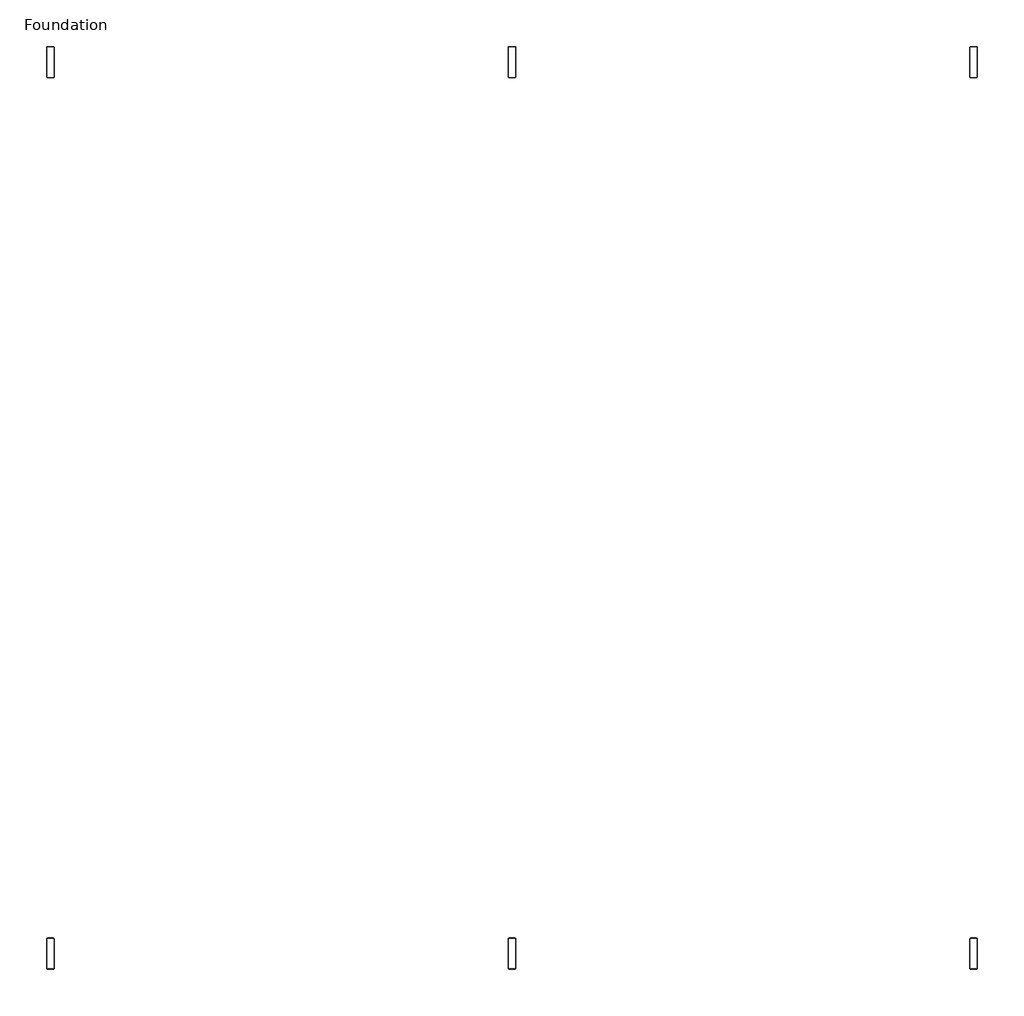
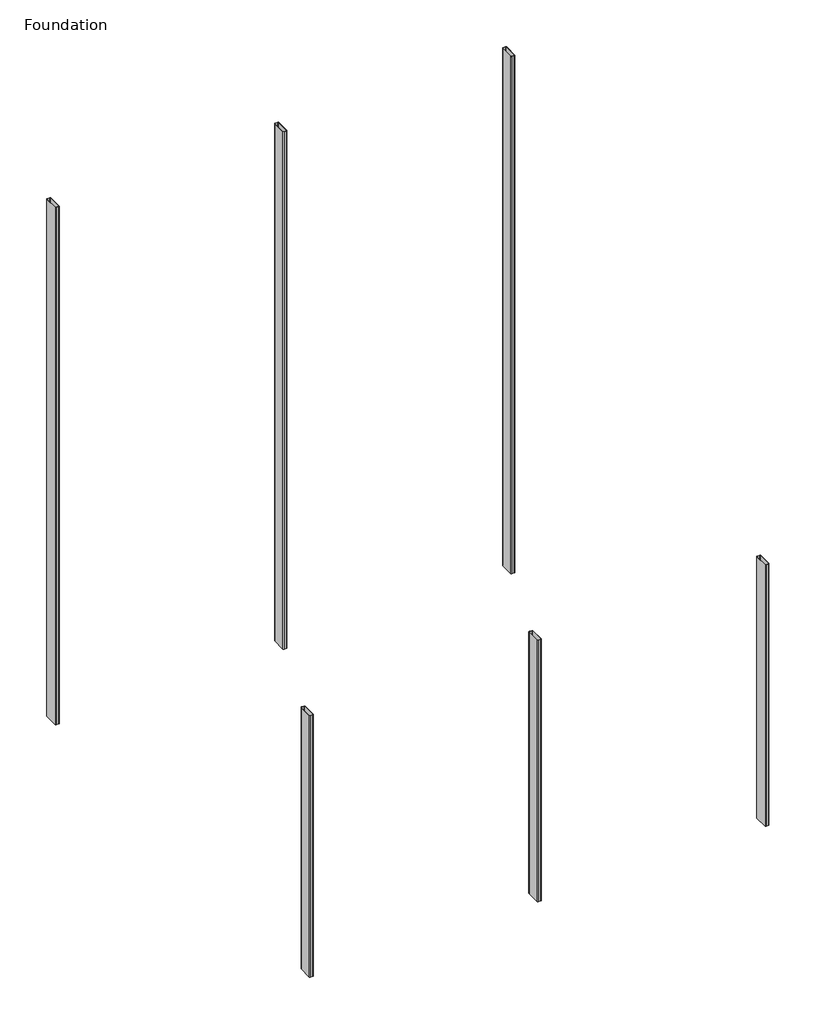
# One storey: 6 columns.
"""IFC4 building model written with IfcOpenShell, lengths in millimetres."""

import ifcopenshell
import ifcopenshell.guid

model = None  # the IFC model being written
_history = None  # IfcOwnerHistory: only IFC2X3 demands one
_inside = {}  # id of a spatial element -> (the spatial element, [elements in it])
_under = {}  # id of a project, library or spatial element -> (it, [spatial elements below it])
_declared = {}  # id of a project -> (the project, [libraries it declares])
_typed = {}  # id of a type object -> (the type object, [elements of that type])
_made_of = {}  # id of a material, layer set ... -> (it, [elements and type objects made of it])


def new_model(schema):
    """Start an empty IFC model of exactly this schema.

    Asked for "IFC4X3", IfcOpenShell would pick the latest addendum, in which some entities
    have other attributes; the version numbers below select the first issue.
    IFC2X3 requires an IfcOwnerHistory on every rooted entity: one is made here for all.
    """
    global model, _history
    if schema == "IFC4X3":
        model = ifcopenshell.file(schema_version=(4, 3, 0, 0))
    else:
        model = ifcopenshell.file(schema=schema)
    _inside.clear()
    _under.clear()
    _declared.clear()
    _typed.clear()
    _made_of.clear()
    _history = None
    if model.schema == "IFC2X3":
        org = make("IfcOrganization", Name="unknown")
        user = make(
            "IfcPersonAndOrganization",
            ThePerson=make("IfcPerson", FamilyName="unknown"),
            TheOrganization=org,
        )
        app = make(
            "IfcApplication",
            ApplicationDeveloper=org,
            Version="unknown",
            ApplicationFullName="unknown",
            ApplicationIdentifier="unknown",
        )
        _history = make(
            "IfcOwnerHistory",
            OwningUser=user,
            OwningApplication=app,
            ChangeAction="ADDED",
            CreationDate=0,
        )
    return model


def make(cls, **values):
    """One entity of the class cls with the attributes given. An attribute that is None is left unset."""
    return model.create_entity(
        cls, **{name: value for name, value in values.items() if value is not None}
    )


def rooted(cls, **values):
    """An entity with a GlobalId (a new one), such as an element, a storey or a relation."""
    return make(cls, GlobalId=ifcopenshell.guid.new(), OwnerHistory=_history, **values)


def si_unit(unit_type, name, prefix=None):
    """IfcSIUnit, for example si_unit("LENGTHUNIT", "METRE", prefix="MILLI")."""
    return make("IfcSIUnit", UnitType=unit_type, Prefix=prefix, Name=name)


def assignment(units):
    """IfcUnitAssignment: the units of a project."""
    return None if units is None else make("IfcUnitAssignment", Units=units)


def point(xyz):
    """IfcCartesianPoint."""
    return None if xyz is None else make("IfcCartesianPoint", Coordinates=xyz)


def direction(xyz):
    """IfcDirection."""
    return None if xyz is None else make("IfcDirection", DirectionRatios=xyz)


def frame(location, z_axis=None, x_axis=None):
    """IfcAxis2Placement3D, a coordinate frame: its origin and axes. An axis left out is left unset."""
    return make(
        "IfcAxis2Placement3D",
        Location=point(location),
        Axis=direction(z_axis),
        RefDirection=direction(x_axis),
    )


def frame_2d(location, x_axis=None):
    """IfcAxis2Placement2D, a coordinate frame in the plane: its origin and x axis."""
    return make(
        "IfcAxis2Placement2D", Location=point(location), RefDirection=direction(x_axis)
    )


def origin():
    """The frame at (0, 0, 0) with its axes left unset."""
    return frame((0.0, 0.0, 0.0))


def place(relative_to, where):
    """IfcLocalPlacement: puts the frame where relative to a parent placement (None: the world)."""
    return make(
        "IfcLocalPlacement", PlacementRelTo=relative_to, RelativePlacement=where
    )


def context(
    kind, dimensions, precision=None, world=None, true_north=None, identifier=None
):
    """IfcGeometricRepresentationContext, for example the 3D "Model" context."""
    return make(
        "IfcGeometricRepresentationContext",
        ContextIdentifier=identifier,
        ContextType=kind,
        CoordinateSpaceDimension=dimensions,
        Precision=precision,
        WorldCoordinateSystem=world,
        TrueNorth=true_north,
    )


def project(units=None, contexts=None):
    """IfcProject with its units and contexts."""
    return rooted(
        "IfcProject",
        Name="project",
        RepresentationContexts=contexts,
        UnitsInContext=assignment(units),
    )


def spatial(cls, under=None, at=None, **own):
    """A site, building, storey or space (cls), placed at a placement, below another one or the project."""
    s = rooted(cls, ObjectPlacement=at, **own)
    if under is not None:
        _under.setdefault(under.id(), (under, []))[1].append(s)
    return s


def polyline(points):
    """IfcPolyline through the points."""
    return make("IfcPolyline", Points=[point(p) for p in points])


def circle_curve(where, radius):
    """IfcCircle in the frame where."""
    return make("IfcCircle", Position=where, Radius=radius)


def trimmed(basis, trim1, trim2, sense, master):
    """IfcTrimmedCurve: the piece of a basis curve between two trims."""
    return make(
        "IfcTrimmedCurve",
        BasisCurve=basis,
        Trim1=trim1,
        Trim2=trim2,
        SenseAgreement=sense,
        MasterRepresentation=master,
    )


def segment(curve, same_sense, transition):
    """IfcCompositeCurveSegment."""
    return make(
        "IfcCompositeCurveSegment",
        Transition=transition,
        SameSense=same_sense,
        ParentCurve=curve,
    )


def composite_curve(segments, self_intersect=None):
    """IfcCompositeCurve: segments joined end to end."""
    return make("IfcCompositeCurve", Segments=segments, SelfIntersect=self_intersect)


def outline(outer, holes=None, kind="AREA"):
    """IfcArbitraryClosedProfileDef: a profile drawn as a closed curve; with holes, ...WithVoids."""
    if holes is None:
        return make("IfcArbitraryClosedProfileDef", ProfileType=kind, OuterCurve=outer)
    return make(
        "IfcArbitraryProfileDefWithVoids",
        ProfileType=kind,
        OuterCurve=outer,
        InnerCurves=holes,
    )


def extrude(swept, where, along, depth):
    """IfcExtrudedAreaSolid: the profile swept, set in the frame where, extruded along a direction by depth."""
    return make(
        "IfcExtrudedAreaSolid",
        SweptArea=swept,
        Position=where,
        ExtrudedDirection=direction(along),
        Depth=depth,
    )


def shape(context_of_items, identifier, shape_type, items):
    """IfcShapeRepresentation: the items that make up one representation, for example the "Body"."""
    return make(
        "IfcShapeRepresentation",
        ContextOfItems=context_of_items,
        RepresentationIdentifier=identifier,
        RepresentationType=shape_type,
        Items=items,
    )


def source(mapping_origin, context_of_items, identifier, shape_type, items):
    """IfcRepresentationMap: a shape defined once, which mapped items show again and again."""
    return make(
        "IfcRepresentationMap",
        MappingOrigin=mapping_origin,
        MappedRepresentation=shape(context_of_items, identifier, shape_type, items),
    )


def transform(
    local_origin,
    x_axis=None,
    y_axis=None,
    z_axis=None,
    scale=None,
    scale2=None,
    scale3=None,
    uniform=True,
):
    """IfcCartesianTransformationOperator3D, or its non-uniform kind. x_axis, y_axis, z_axis: its Axis1, 2, 3."""
    if uniform:
        return make(
            "IfcCartesianTransformationOperator3D",
            Axis1=direction(x_axis),
            Axis2=direction(y_axis),
            LocalOrigin=point(local_origin),
            Scale=scale,
            Axis3=direction(z_axis),
        )
    return make(
        "IfcCartesianTransformationOperator3DnonUniform",
        Axis1=direction(x_axis),
        Axis2=direction(y_axis),
        LocalOrigin=point(local_origin),
        Scale=scale,
        Axis3=direction(z_axis),
        Scale2=scale2,
        Scale3=scale3,
    )


def mapped(mapping_source, mapping_target):
    """IfcMappedItem: shows the shape of a source again, moved by a transform."""
    return make(
        "IfcMappedItem", MappingSource=mapping_source, MappingTarget=mapping_target
    )


def made_of(thing, what):
    """Note that an element or type object is made of a material, layer set ...; save() writes the relation."""
    if what is not None:
        _made_of.setdefault(what.id(), (what, []))[1].append(thing)
    return thing


def element(
    cls,
    number,
    at=None,
    inside=None,
    cuts=None,
    type_object=None,
    material=None,
    context=None,
    identifier="Body",
    shape_type=None,
    held_by="IfcProductDefinitionShape",
    body=None,
    shapes=None,
    **own,
):
    """One element of the class cls, such as IfcWall. Its Tag is "e" and its number.

    at: its placement. inside: the storey or other place that contains it. cuts: it is an
    opening in that element (IfcRelVoidsElement). A single representation is given by context,
    identifier, shape_type and body (its items); several are given by shapes. held_by: the class
    of the entity that holds the representations. save() writes the other relations.
    """
    e = rooted(cls, Tag="e%d" % number, ObjectPlacement=at, **own)
    if body is not None:
        shapes = [shape(context, identifier, shape_type, body)]
    if shapes is not None:
        e.Representation = make(held_by, Representations=shapes)
    if inside is not None:
        _inside.setdefault(inside.id(), (inside, []))[1].append(e)
    if cuts is not None:
        rooted(
            "IfcRelVoidsElement", RelatingBuildingElement=cuts, RelatedOpeningElement=e
        )
    if type_object is not None:
        _typed.setdefault(type_object.id(), (type_object, []))[1].append(e)
    return made_of(e, material)


def aggregate(whole, parts):
    """IfcRelAggregates: a whole, such as a stair, and the parts it consists of."""
    return rooted("IfcRelAggregates", RelatingObject=whole, RelatedObjects=parts)


def save(model, path):
    """Write the relations noted so far, then the file.

    IfcRelAggregates (storeys below a building ...), IfcRelContainedInSpatialStructure (elements
    in a storey), IfcRelDefinesByType, IfcRelAssociatesMaterial and IfcRelDeclares: one each for
    every whole, place, type object, material and project.
    """
    for whole, parts in _under.values():
        aggregate(whole, parts)
    for where, things in _inside.values():
        rooted(
            "IfcRelContainedInSpatialStructure",
            RelatedElements=things,
            RelatingStructure=where,
        )
    for kind, things in _typed.values():
        rooted("IfcRelDefinesByType", RelatedObjects=things, RelatingType=kind)
    for what, things in _made_of.values():
        rooted("IfcRelAssociatesMaterial", RelatedObjects=things, RelatingMaterial=what)
    for by, libraries in _declared.values():
        rooted("IfcRelDeclares", RelatingContext=by, RelatedDefinitions=libraries)
    model.write(path)


def hss_hollow_structural_section_column_hss8x2x3_16_e881e9b5(model_context):
    return source(origin(), model_context, "Body", "SweptSolid", [
        extrude(outline(composite_curve([segment(trimmed(circle_curve(frame_2d((16.5608, 92.7608)), 8.8392), [point((16.5608, 101.6))], [point((25.4, 92.7608))], False, "CARTESIAN"), True, "CONTINUOUS"), segment(polyline([(25.4, 92.7608), (25.4, -92.7608)]), True, "CONTINUOUS"), segment(trimmed(circle_curve(frame_2d((16.5608, -92.7608)), 8.8392), [point((25.4, -92.7608))], [point((16.5608, -101.6))], False, "CARTESIAN"), True, "CONTINUOUS"), segment(polyline([(16.5608, -101.6), (-16.5608, -101.6)]), True, "CONTINUOUS"), segment(trimmed(circle_curve(frame_2d((-16.5608, -92.7608)), 8.8392), [point((-16.5608, -101.6))], [point((-25.4, -92.7608))], False, "CARTESIAN"), True, "CONTINUOUS"), segment(polyline([(-25.4, -92.7608), (-25.4, 92.7608)]), True, "CONTINUOUS"), segment(trimmed(circle_curve(frame_2d((-16.5608, 92.7608)), 8.8392), [point((-25.4, 92.7608))], [point((-16.5608, 101.6))], False, "CARTESIAN"), True, "CONTINUOUS"), segment(polyline([(-16.5608, 101.6), (16.5608, 101.6)]), True, "CONTINUOUS")], self_intersect=False), holes=[composite_curve([segment(polyline([(16.5608, 97.1804), (-16.5608, 97.1804)]), True, "CONTINUOUS"), segment(trimmed(circle_curve(frame_2d((-16.5608, 92.7608)), 4.4196), [point((-16.5608, 97.1804))], [point((-20.9804, 92.7608))], True, "CARTESIAN"), True, "CONTINUOUS"), segment(polyline([(-20.9804, 92.7608), (-20.9804, -92.7608)]), True, "CONTINUOUS"), segment(trimmed(circle_curve(frame_2d((-16.5608, -92.7608)), 4.4196), [point((-20.9804, -92.7608))], [point((-16.5608, -97.1804))], True, "CARTESIAN"), True, "CONTINUOUS"), segment(polyline([(-16.5608, -97.1804), (16.5608, -97.1804)]), True, "CONTINUOUS"), segment(trimmed(circle_curve(frame_2d((16.5608, -92.7608)), 4.4196), [point((16.5608, -97.1804))], [point((20.9804, -92.7608))], True, "CARTESIAN"), True, "CONTINUOUS"), segment(polyline([(20.9804, -92.7608), (20.9804, 92.7608)]), True, "CONTINUOUS"), segment(trimmed(circle_curve(frame_2d((16.5608, 92.7608)), 4.4196), [point((20.9804, 92.7608))], [point((16.5608, 97.1804))], True, "CARTESIAN"), True, "CONTINUOUS")], self_intersect=False)]), frame((0.0, 0.0, -1200.0), z_axis=(0.0, 0.0, 1.0), x_axis=(1.0, 0.0, 0.0)), (0.0, 0.0, 1.0), 7200.0),
    ])


def hss_hollow_structural_section_column_hss8x2x3_16_13fa7c93(model_context):
    return source(origin(), model_context, "Body", "SweptSolid", [
        extrude(outline(composite_curve([segment(trimmed(circle_curve(frame_2d((16.5608, 92.7608)), 8.8392), [point((16.5608, 101.6))], [point((25.4, 92.7608))], False, "CARTESIAN"), True, "CONTINUOUS"), segment(polyline([(25.4, 92.7608), (25.4, -92.7608)]), True, "CONTINUOUS"), segment(trimmed(circle_curve(frame_2d((16.5608, -92.7608)), 8.8392), [point((25.4, -92.7608))], [point((16.5608, -101.6))], False, "CARTESIAN"), True, "CONTINUOUS"), segment(polyline([(16.5608, -101.6), (-16.5608, -101.6)]), True, "CONTINUOUS"), segment(trimmed(circle_curve(frame_2d((-16.5608, -92.7608)), 8.8392), [point((-16.5608, -101.6))], [point((-25.4, -92.7608))], False, "CARTESIAN"), True, "CONTINUOUS"), segment(polyline([(-25.4, -92.7608), (-25.4, 92.7608)]), True, "CONTINUOUS"), segment(trimmed(circle_curve(frame_2d((-16.5608, 92.7608)), 8.8392), [point((-25.4, 92.7608))], [point((-16.5608, 101.6))], False, "CARTESIAN"), True, "CONTINUOUS"), segment(polyline([(-16.5608, 101.6), (16.5608, 101.6)]), True, "CONTINUOUS")], self_intersect=False), holes=[composite_curve([segment(polyline([(16.5608, 97.1804), (-16.5608, 97.1804)]), True, "CONTINUOUS"), segment(trimmed(circle_curve(frame_2d((-16.5608, 92.7608)), 4.4196), [point((-16.5608, 97.1804))], [point((-20.9804, 92.7608))], True, "CARTESIAN"), True, "CONTINUOUS"), segment(polyline([(-20.9804, 92.7608), (-20.9804, -92.7608)]), True, "CONTINUOUS"), segment(trimmed(circle_curve(frame_2d((-16.5608, -92.7608)), 4.4196), [point((-20.9804, -92.7608))], [point((-16.5608, -97.1804))], True, "CARTESIAN"), True, "CONTINUOUS"), segment(polyline([(-16.5608, -97.1804), (16.5608, -97.1804)]), True, "CONTINUOUS"), segment(trimmed(circle_curve(frame_2d((16.5608, -92.7608)), 4.4196), [point((16.5608, -97.1804))], [point((20.9804, -92.7608))], True, "CARTESIAN"), True, "CONTINUOUS"), segment(polyline([(20.9804, -92.7608), (20.9804, 92.7608)]), True, "CONTINUOUS"), segment(trimmed(circle_curve(frame_2d((16.5608, 92.7608)), 4.4196), [point((20.9804, 92.7608))], [point((16.5608, 97.1804))], True, "CARTESIAN"), True, "CONTINUOUS")], self_intersect=False)]), frame((0.0, 0.0, -1200.0), z_axis=(0.0, 0.0, 1.0), x_axis=(1.0, 0.0, 0.0)), (0.0, 0.0, 1.0), 3639.0),
    ])


model = new_model("IFC4")

# Units and contexts
model_context = context("Model", 3, world=origin())
ifc_project = project(units=[si_unit("LENGTHUNIT", "METRE", prefix="MILLI")], contexts=[model_context])

# Site, building, storey
site = spatial("IfcSite", under=ifc_project)
building = spatial("IfcBuilding", under=site)
storey = spatial("IfcBuildingStorey", under=building, Name="Foundation", Elevation=-1200.0)

# Columns
placement = place(None, origin())
hss_hollow_structural_section_column_hss8x2x3_16_shape = hss_hollow_structural_section_column_hss8x2x3_16_e881e9b5(model_context)
element("IfcColumn", 1, ObjectType="HSS-Hollow Structural Section-Column : HSS8X2X3/16", at=placement, inside=storey, context=model_context, shape_type="MappedRepresentation", body=[
    mapped(hss_hollow_structural_section_column_hss8x2x3_16_shape, transform((13061.9315174, 2696.9060214, 0.0), x_axis=(-1.0, 0.0, 0.0), y_axis=(0.0, -1.0, 0.0), z_axis=(0.0, 0.0, 1.0))),
])
element("IfcColumn", 2, ObjectType="HSS-Hollow Structural Section-Column : HSS8X2X3/16", at=placement, inside=storey, context=model_context, shape_type="MappedRepresentation", body=[
    mapped(hss_hollow_structural_section_column_hss8x2x3_16_shape, transform((10061.9315174, 2696.9060214, 0.0), x_axis=(-1.0, 0.0, 0.0), y_axis=(0.0, -1.0, 0.0), z_axis=(0.0, 0.0, 1.0))),
])
element("IfcColumn", 3, ObjectType="HSS-Hollow Structural Section-Column : HSS8X2X3/16", at=placement, inside=storey, context=model_context, shape_type="MappedRepresentation", body=[
    mapped(hss_hollow_structural_section_column_hss8x2x3_16_shape, transform((7061.9315174, 2696.9060214, 0.0), x_axis=(-1.0, 0.0, 0.0), y_axis=(0.0, -1.0, 0.0), z_axis=(0.0, 0.0, 1.0))),
])
hss_hollow_structural_section_column_hss8x2x3_16_2_shape = hss_hollow_structural_section_column_hss8x2x3_16_13fa7c93(model_context)
element("IfcColumn", 4, ObjectType="HSS-Hollow Structural Section-Column : HSS8X2X3/16", at=placement, inside=storey, context=model_context, shape_type="MappedRepresentation", body=[
    mapped(hss_hollow_structural_section_column_hss8x2x3_16_2_shape, transform((13061.9315174, -3100.0939786, 0.0), x_axis=(-1.0, 0.0, 0.0), y_axis=(0.0, -1.0, 0.0), z_axis=(0.0, 0.0, 1.0))),
])
element("IfcColumn", 5, ObjectType="HSS-Hollow Structural Section-Column : HSS8X2X3/16", at=placement, inside=storey, context=model_context, shape_type="MappedRepresentation", body=[
    mapped(hss_hollow_structural_section_column_hss8x2x3_16_2_shape, transform((10061.9315174, -3100.0939786, 0.0), x_axis=(-1.0, 0.0, 0.0), y_axis=(0.0, -1.0, 0.0), z_axis=(0.0, 0.0, 1.0))),
])
element("IfcColumn", 6, ObjectType="HSS-Hollow Structural Section-Column : HSS8X2X3/16", at=placement, inside=storey, context=model_context, shape_type="MappedRepresentation", body=[
    mapped(hss_hollow_structural_section_column_hss8x2x3_16_2_shape, transform((7061.9315174, -3100.0939786, 0.0), x_axis=(-1.0, 0.0, 0.0), y_axis=(0.0, -1.0, 0.0), z_axis=(0.0, 0.0, 1.0))),
])

save(model, "model.ifc")

# Revit data of these elements
# Project information
#   Project Issue Date = "Issue Date"
#   Project Status = "Project Status"
#   Client Name = "Owner"
#   Project Address = "Enter address here"
#   Project Name = "Project Name"
#   Project Number = "0001"
# Type "HSS-Hollow Structural Section-Column : HSS8X2X3/16"
#   Assembly Code = "B10"
#   Shape = "Rect."
#   Cost = 1
#   W = 12
#   Ht = 203.2 mm
#   b = 50.8 mm
#   kr = 8.839 mm
#   t = 4.42 mm
#   A = 0.00211612 m²
#   Structural Material [instance default] = Steel ASTM A500, Grade B, Rectangular and Square
# Elements 1, 2, 3, 4, 5, 6 (IfcColumn, "HSS-Hollow Structural Section-Column : HSS8X2X3/16")
#   Structural Material = Metal - Steel 43-275
#   Phase Created = New Construction
#   Materials on its faces: "Metal - Steel 43-275"
# Materials
#   "Steel ASTM A500, Grade B, Rectangular and Square": class "Metal", colour RGB 199 199 199, transparency 0, Description = "Carbon steel", Cost = 0
#   "Metal - Steel 43-275": class "Metal", colour RGB 247 247 247, transparency 0, Cost = 0
